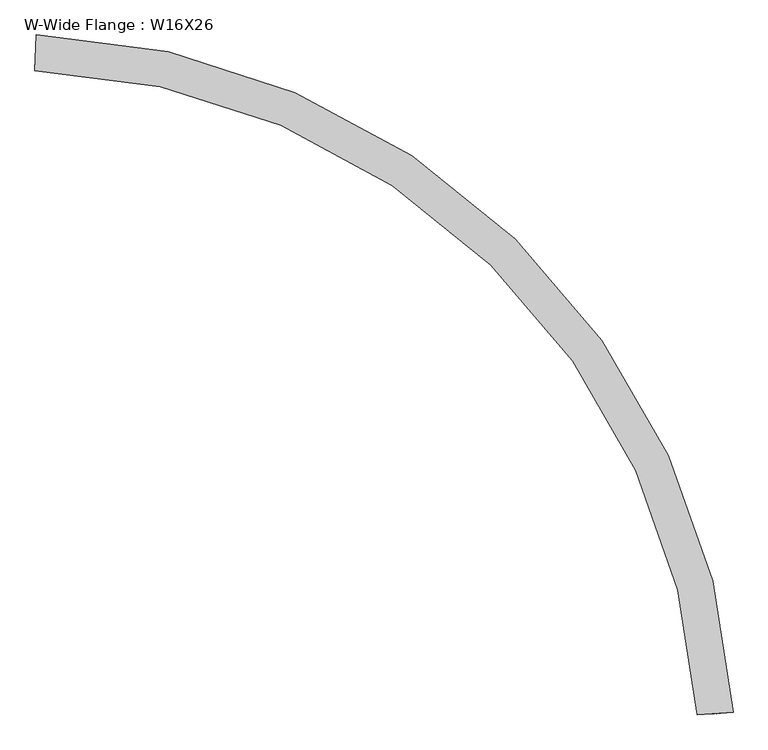
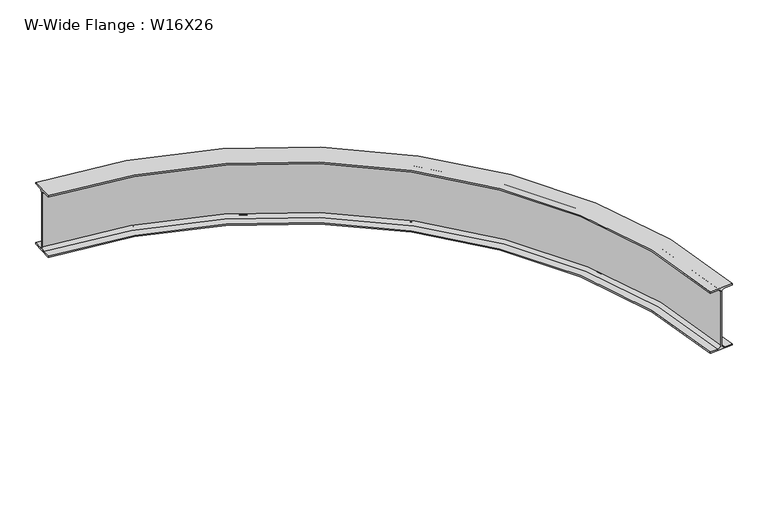
"""IFC4 building model written with IfcOpenShell, lengths in millimetres: beam geometry, W-Wide Flange : W16X26."""

from ifc_helpers import new_model, si_unit, point, frame, origin, place, context, project, spatial, polyline, circle_curve, ellipse_curve, trimmed, source, transform, mapped, element, save
from ifc_brep_helpers import plane_surface, cylinder_surface, revolved_surface, advanced_brep


def w_wide_flange_w16x26_7959fbc0(model_context):
    return source(origin(), model_context, "Body", "AdvancedBrep", [
        advanced_brep(
        [(2687.1196296, -2593.7096303, -190.5496094), (2687.1196296, -2593.7096303, -199.2808594), (2826.5456481, -2584.9646111, -199.2808594), (2826.5456481, -2584.9646111, -190.5496094), (2778.2218576, -2587.9955553, -190.5496094), (2760.001412, -2589.1383703, -172.2933594), (2760.001412, -2589.1383703, 172.2933594), (2778.2218576, -2587.9955553, 190.5496094), (2826.5456481, -2584.9646111, 190.5496094), (2826.5456481, -2584.9646111, 199.2808594), (2687.1196296, -2593.7096303, 199.2808594), (2687.1196296, -2593.7096303, 190.5496094), (2735.4434201, -2590.6786861, 190.5496094), (2753.6638657, -2589.5358711, 172.2933594), (2753.6638657, -2589.5358711, -172.2933594), (2735.4434201, -2590.6786861, -190.5496094), (94.7733091, -71.5185418, -190.5496094), (96.477664, -23.1297981, -190.5496094), (97.1202896, -4.8848619, -172.2933594), (97.1202896, -4.8848619, 172.2933594), (96.477664, -23.1297981, 190.5496094), (94.7733091, -71.5185418, 190.5496094), (94.7733091, -71.5185418, 199.2808594), (99.6907921, 68.0948829, 199.2808594), (99.6907921, 68.0948829, 190.5496094), (97.9864372, 19.7061391, 190.5496094), (97.3438116, 1.4612029, 172.2933594), (97.3438116, 1.4612029, -172.2933594), (97.9864372, 19.7061391, -190.5496094), (99.6907921, 68.0948829, -190.5496094), (99.6907921, 68.0948829, -199.2808594), (94.7733091, -71.5185418, -199.2808594)],
        [
            (0, 1),
            (1, 2),
            (2, 3),
            (3, 4),
            (4, 5, circle_curve(frame((2778.2218576, -2587.9955553, -172.2933594), z_axis=(-0.06259856251271431, 0.9980387868070768, 0.0), x_axis=(0.9980387868070768, 0.06259856251271431, 0.0)), 18.25625)),
            (5, 6),
            (6, 7, circle_curve(frame((2778.2218576, -2587.9955553, 172.2933594), z_axis=(-0.06259856251271431, 0.9980387868070768, 0.0), x_axis=(0.9980387868070768, 0.06259856251271431, 0.0)), 18.25625)),
            (7, 8),
            (8, 9),
            (9, 10),
            (10, 11),
            (11, 12),
            (12, 13, circle_curve(frame((2735.4434201, -2590.6786861, 172.2933594), z_axis=(-0.06259856251271431, 0.9980387868070768, 0.0), x_axis=(0.9980387868070768, 0.06259856251271431, 0.0)), 18.25625)),
            (13, 14),
            (14, 15, circle_curve(frame((2735.4434201, -2590.6786861, -172.2933594), z_axis=(-0.06259856251271431, 0.9980387868070768, 0.0), x_axis=(0.9980387868070768, 0.06259856251271431, 0.0)), 18.25625)),
            (15, 0),
            (16, 17),
            (17, 18, circle_curve(frame((96.477664, -23.1297981, -172.2933594), z_axis=(0.9993802771321465, -0.035200307942887296, 0.0), x_axis=(0.035200307942887296, 0.9993802771321465, 0.0)), 18.25625)),
            (18, 19),
            (19, 20, circle_curve(frame((96.477664, -23.1297981, 172.2933594), z_axis=(0.9993802771321465, -0.035200307942887296, 0.0), x_axis=(0.035200307942887296, 0.9993802771321465, 0.0)), 18.25625)),
            (20, 21),
            (21, 22),
            (22, 23),
            (23, 24),
            (24, 25),
            (25, 26, circle_curve(frame((97.9864372, 19.7061391, 172.2933594), z_axis=(0.9993802771321465, -0.035200307942887296, 0.0), x_axis=(0.035200307942887296, 0.9993802771321465, 0.0)), 18.25625)),
            (26, 27),
            (27, 28, circle_curve(frame((97.9864372, 19.7061391, -172.2933594), z_axis=(0.9993802771321465, -0.035200307942887296, 0.0), x_axis=(0.035200307942887296, 0.9993802771321465, 0.0)), 18.25625)),
            (28, 29),
            (29, 30),
            (30, 31),
            (31, 16),
            (15, 17, circle_curve(frame((0.0, -2762.25, -190.5496094), z_axis=(0.0, 0.0, 1.0), x_axis=(-1.0, 0.0, 0.0)), 2740.81875)),
            (16, 0, circle_curve(frame((0.0, -2762.25, -190.5496094), z_axis=(0.0, 0.0, -1.0), x_axis=(-1.0, 0.0, 0.0)), 2692.4)),
            (14, 18, circle_curve(frame((0.0, -2762.25, -172.2933594), z_axis=(0.0, 0.0, 1.0), x_axis=(-1.0, 0.0, 0.0)), 2759.075)),
            (13, 19, circle_curve(frame((0.0, -2762.25, 172.2933594), z_axis=(0.0, 0.0, 1.0), x_axis=(-1.0, 0.0, 0.0)), 2759.075)),
            (12, 20, circle_curve(frame((0.0, -2762.25, 190.5496094), z_axis=(0.0, 0.0, 1.0), x_axis=(-1.0, 0.0, 0.0)), 2740.81875)),
            (11, 21, circle_curve(frame((0.0, -2762.25, 190.5496094), z_axis=(0.0, 0.0, 1.0), x_axis=(-1.0, 0.0, 0.0)), 2692.4)),
            (10, 22, circle_curve(frame((0.0, -2762.25, 199.2808594), z_axis=(0.0, 0.0, 1.0), x_axis=(-1.0, 0.0, 0.0)), 2692.4)),
            (9, 23, circle_curve(frame((0.0, -2762.25, 199.2808594), z_axis=(0.0, 0.0, 1.0), x_axis=(-1.0, 0.0, 0.0)), 2832.1)),
            (8, 24, circle_curve(frame((0.0, -2762.25, 190.5496094), z_axis=(0.0, 0.0, 1.0), x_axis=(-1.0, 0.0, 0.0)), 2832.1)),
            (7, 25, circle_curve(frame((0.0, -2762.25, 190.5496094), z_axis=(0.0, 0.0, 1.0), x_axis=(-1.0, 0.0, 0.0)), 2783.68125)),
            (6, 26, circle_curve(frame((0.0, -2762.25, 172.2933594), z_axis=(0.0, 0.0, 1.0), x_axis=(-1.0, 0.0, 0.0)), 2765.425)),
            (5, 27, circle_curve(frame((0.0, -2762.25, -172.2933594), z_axis=(0.0, 0.0, 1.0), x_axis=(-1.0, 0.0, 0.0)), 2765.425)),
            (4, 28, circle_curve(frame((0.0, -2762.25, -190.5496094), z_axis=(0.0, 0.0, 1.0), x_axis=(-1.0, 0.0, 0.0)), 2783.68125)),
            (3, 29, circle_curve(frame((0.0, -2762.25, -190.5496094), z_axis=(0.0, 0.0, 1.0), x_axis=(-1.0, 0.0, 0.0)), 2832.1)),
            (2, 30, circle_curve(frame((0.0, -2762.25, -199.2808594), z_axis=(0.0, 0.0, 1.0), x_axis=(-1.0, 0.0, 0.0)), 2832.1)),
            (1, 31, circle_curve(frame((0.0, -2762.25, -199.2808594), z_axis=(0.0, 0.0, 1.0), x_axis=(-1.0, 0.0, 0.0)), 2692.4)),
        ],
        [
            plane_surface(frame((2756.8326389, -2589.3371207, 0.0), z_axis=(0.06259856251270805, -0.9980387868070772, 0.0), x_axis=(0.0, 0.0, 1.0))),
            plane_surface(frame((97.2320506, -1.7118295, 0.0), z_axis=(-0.9993802771321463, 0.03520030794289379, 0.0), x_axis=(0.0, 0.0, 1.0))),
            plane_surface(frame((0.0, -2762.25, -190.5496094), z_axis=(0.0, 0.0, 1.0), x_axis=(-1.0, 0.0, 0.0))),
            revolved_surface(trimmed(ellipse_curve(frame((-2740.81875, -2762.25, -172.2933594), z_axis=(0.0, -1.0, 0.0), x_axis=(-1.0, 0.0, 0.0)), 18.25625, 18.25625), [point((-2759.075, -2762.25, -172.2933594))], [point((-2740.81875, -2762.25, -190.5496094))], True, "CARTESIAN"), (0.0, -2762.25, 0.0), (0.0, 0.0, 1.0)),
            revolved_surface(polyline([(-2759.075, -2762.25, 172.2933594), (-2759.075, -2762.25, -172.2933594)]), (0.0, -2762.25, 0.0), (0.0, 0.0, 1.0)),
            revolved_surface(trimmed(ellipse_curve(frame((-2740.81875, -2762.25, 172.2933594), z_axis=(0.0, -1.0, 0.0), x_axis=(-1.0, 0.0, 0.0)), 18.25625, 18.25625), [point((-2740.81875, -2762.25, 190.5496094))], [point((-2759.075, -2762.25, 172.2933594))], True, "CARTESIAN"), (0.0, -2762.25, 0.0), (0.0, 0.0, 1.0)),
            plane_surface(frame((0.0, -2762.25, 190.5496094), z_axis=(0.0, 0.0, -1.0), x_axis=(-1.0, 0.0, 0.0))),
            revolved_surface(polyline([(-2692.4, -2762.25, 199.2808594), (-2692.4, -2762.25, 190.5496094)]), (0.0, -2762.25, 0.0), (0.0, 0.0, 1.0)),
            plane_surface(frame((0.0, -2762.25, 199.2808594), z_axis=(0.0, 0.0, 1.0), x_axis=(-1.0, 0.0, 0.0))),
            cylinder_surface(frame((0.0, -2762.25, 0.0), z_axis=(0.0, 0.0, 1.0), x_axis=(-1.0, 0.0, 0.0)), 2832.1),
            revolved_surface(trimmed(ellipse_curve(frame((-2783.68125, -2762.25, 172.2933594), z_axis=(0.0, -1.0, 0.0), x_axis=(-1.0, 0.0, 0.0)), 18.25625, 18.25625), [point((-2765.425, -2762.25, 172.2933594))], [point((-2783.68125, -2762.25, 190.5496094))], True, "CARTESIAN"), (0.0, -2762.25, 0.0), (0.0, 0.0, 1.0)),
            cylinder_surface(frame((0.0, -2762.25, 0.0), z_axis=(0.0, 0.0, 1.0), x_axis=(-1.0, 0.0, 0.0)), 2765.425),
            revolved_surface(trimmed(ellipse_curve(frame((-2783.68125, -2762.25, -172.2933594), z_axis=(0.0, -1.0, 0.0), x_axis=(-1.0, 0.0, 0.0)), 18.25625, 18.25625), [point((-2783.68125, -2762.25, -190.5496094))], [point((-2765.425, -2762.25, -172.2933594))], True, "CARTESIAN"), (0.0, -2762.25, 0.0), (0.0, 0.0, 1.0)),
            plane_surface(frame((0.0, -2762.25, -199.2808594), z_axis=(0.0, 0.0, -1.0), x_axis=(-1.0, 0.0, 0.0))),
            revolved_surface(polyline([(-2692.4, -2762.25, -190.5496094), (-2692.4, -2762.25, -199.2808594)]), (0.0, -2762.25, 0.0), (0.0, 0.0, 1.0)),
        ],
        [
            (0, [[1, 2, 3, 4, 5, 6, 7, 8, 9, 10, 11, 12, 13, 14, 15, 16]]),
            (1, [[17, 18, 19, 20, 21, 22, 23, 24, 25, 26, 27, 28, 29, 30, 31, 32]]),
            (2, [[33, -17, 34, -16]]),
            (3, [[35, -18, -33, -15]]),
            (4, [[36, -19, -35, -14]]),
            (5, [[37, -20, -36, -13]]),
            (6, [[38, -21, -37, -12]]),
            (7, [[39, -22, -38, -11]]),
            (8, [[40, -23, -39, -10]]),
            (9, [[41, -24, -40, -9]]),
            (6, [[42, -25, -41, -8]]),
            (10, [[43, -26, -42, -7]]),
            (11, [[44, -27, -43, -6]]),
            (12, [[45, -28, -44, -5]]),
            (2, [[46, -29, -45, -4]]),
            (9, [[47, -30, -46, -3]]),
            (13, [[48, -31, -47, -2]]),
            (14, [[-34, -32, -48, -1]]),
        ],
    ),
    ])


if __name__ == "__main__":
    model = new_model("IFC4")
    model_context = context("Model", 3, world=origin())
    ifc_project = project(units=[si_unit("LENGTHUNIT", "METRE", prefix="MILLI")], contexts=[model_context])
    site = spatial("IfcSite", under=ifc_project)
    building = spatial("IfcBuilding", under=site)
    placement = place(None, origin())
    w_wide_flange_w16x26_shape = w_wide_flange_w16x26_7959fbc0(model_context)
    element("IfcBeam", 1, ObjectType="W-Wide Flange : W16X26", at=placement, inside=building, context=model_context, shape_type="MappedRepresentation", body=[
        mapped(w_wide_flange_w16x26_shape, transform((0.0, 0.0, 0.0), x_axis=(1.0, 0.0, 0.0), y_axis=(0.0, 1.0, 0.0), z_axis=(0.0, 0.0, 1.0))),
    ])
    save(model, "model.ifc")

# Revit data of these elements
# Type "W-Wide Flange : W16X26"
#   Assembly Code = "B10"
#   W = 26
#   Start Extension Calculation [instance default] = 10' - 0"
#   Start Extension [instance default] = -0' - 0 1/2"
#   End Extension Calculation [instance default] = 10' - 0"
#   End Extension [instance default] = -0' - 0 1/2"
#   Length [instance default] = 5' - 0"
#   bf = 0' - 5 1/2"
#   d = 1' - 3 177/256"
#   k = 0' - 1 1/16"
#   k2 = 0' - 0 23/32"
#   tf = 0' - 0 11/32"
#   tw = 0' - 0 1/4"
#   A = 0.05 SF
#   Beam Material [instance default] = Metal - Steel - ASTM A992
# Element 1 (IfcBeam, "W-Wide Flange : W16X26")
#   Materials on its faces: "Metal - Steel - ASTM A992"
# Materials
#   "Metal - Steel - ASTM A992": class "Metal", colour RGB 128 0 0, transparency 0
